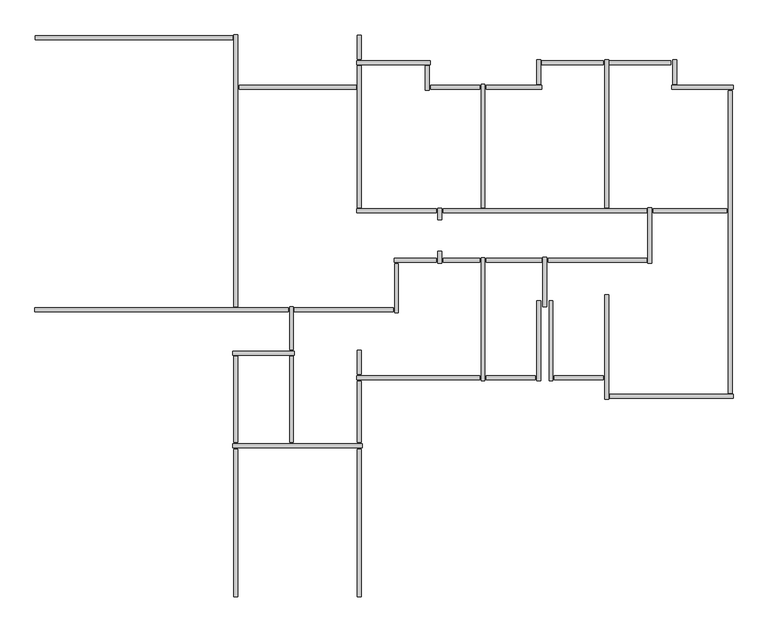
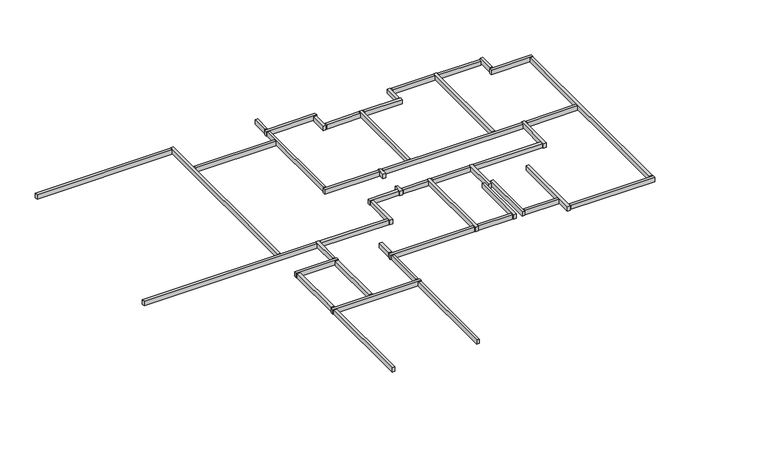
"""IFC4 building model written with IfcOpenShell, lengths in millimetres: beam geometry, Graute viga de respaldo21 : Graute viga de respaldo."""

from ifc_helpers import new_model, si_unit, frame, origin, place, context, project, spatial, polyline, outline, extrude, source, transform, mapped, element, save


def beam_0cd8a0a3(model_context):
    return source(origin(), model_context, "Body", "SweptSolid", [
        extrude(outline(polyline([(-62804.9587292, 72814.9577736), (-62804.9587292, 72720.9577736), (-67594.9587292, 72720.9577736), (-67594.9587292, 72814.9577736), (-62804.9587292, 72814.9577736)])), frame((0.0, 0.0, 17632.9999999), z_axis=(0.0, 0.0, 1.0), x_axis=(1.0, 0.0, 0.0)), (0.0, 0.0, 1.0), 167.0),
        extrude(outline(polyline([(-59771.9587292, 62785.4278788), (-59677.9587292, 62785.4278788), (-59677.9587292, 59195.4278788), (-59771.9587292, 59195.4278788), (-59771.9587292, 62785.4278788)])), frame((0.0, 0.0, 17632.9999999), z_axis=(0.0, 0.0, 1.0), x_axis=(1.0, 0.0, 0.0)), (0.0, 0.0, 1.0), 167.0),
        extrude(outline(polyline([(-62771.9587292, 62785.4278788), (-62677.9587292, 62785.4278788), (-62677.9587292, 59195.4278788), (-62771.9587292, 59195.4278788), (-62771.9587292, 62785.4278788)])), frame((0.0, 0.0, 17632.9999999), z_axis=(0.0, 0.0, 1.0), x_axis=(1.0, 0.0, 0.0)), (0.0, 0.0, 1.0), 167.0),
        extrude(outline(polyline([(-54994.9587292, 64468.4278788), (-54994.9587292, 64562.4278788), (-53804.9587292, 64562.4278788), (-53804.9587292, 64468.4278788), (-54994.9587292, 64468.4278788)])), frame((0.0, 0.0, 17632.9999999), z_axis=(0.0, 0.0, 1.0), x_axis=(1.0, 0.0, 0.0)), (0.0, 0.0, 1.0), 167.0),
        extrude(outline(polyline([(-56644.9587292, 64468.4278788), (-56644.9587292, 64562.4278788), (-55454.9587292, 64562.4278788), (-55454.9587292, 64468.4278788), (-56644.9587292, 64468.4278788)])), frame((0.0, 0.0, 17632.9999999), z_axis=(0.0, 0.0, 1.0), x_axis=(1.0, 0.0, 0.0)), (0.0, 0.0, 1.0), 167.0),
        extrude(outline(polyline([(-52594.9587292, 68518.4278788), (-52594.9587292, 68612.4278788), (-50804.9587292, 68612.4278788), (-50804.9587292, 68518.4278788), (-52594.9587292, 68518.4278788)])), frame((0.0, 0.0, 17632.9999999), z_axis=(0.0, 0.0, 1.0), x_axis=(1.0, 0.0, 0.0)), (0.0, 0.0, 1.0), 167.0),
        extrude(outline(polyline([(-57994.9587292, 71518.4278788), (-57994.9587292, 71612.4278788), (-56804.9587292, 71612.4278788), (-56804.9587292, 71518.4278788), (-57994.9587292, 71518.4278788)])), frame((0.0, 0.0, 17632.9999999), z_axis=(0.0, 0.0, 1.0), x_axis=(1.0, 0.0, 0.0)), (0.0, 0.0, 1.0), 167.0),
        extrude(outline(polyline([(-58027.9587292, 71495.4278788), (-58121.9587292, 71495.4278788), (-58121.9587292, 72085.4278788), (-58027.9587292, 72085.4278788), (-58027.9587292, 71495.4278788)])), frame((0.0, 0.0, 17632.9999999), z_axis=(0.0, 0.0, 1.0), x_axis=(1.0, 0.0, 0.0)), (0.0, 0.0, 1.0), 167.0),
        extrude(outline(polyline([(-59794.9587292, 72118.4278788), (-59794.9587292, 72212.4278788), (-58004.9587292, 72212.4278788), (-58004.9587292, 72118.4278788), (-59794.9587292, 72118.4278788)])), frame((0.0, 0.0, 17632.9999999), z_axis=(0.0, 0.0, 1.0), x_axis=(1.0, 0.0, 0.0)), (0.0, 0.0, 1.0), 167.0),
        extrude(outline(polyline([(-57821.9587292, 68635.4278788), (-57727.9587292, 68635.4278788), (-57727.9587292, 68345.4278788), (-57821.9587292, 68345.4278788), (-57821.9587292, 68635.4278788)])), frame((0.0, 0.0, 17632.9999999), z_axis=(0.0, 0.0, 1.0), x_axis=(1.0, 0.0, 0.0)), (0.0, 0.0, 1.0), 167.0),
        extrude(outline(polyline([(-55144.9587292, 67318.4278788), (-55144.9587292, 67412.4278788), (-52754.9587292, 67412.4278788), (-52754.9587292, 67318.4278788), (-55144.9587292, 67318.4278788)])), frame((0.0, 0.0, 17632.9999999), z_axis=(0.0, 0.0, 1.0), x_axis=(1.0, 0.0, 0.0)), (0.0, 0.0, 1.0), 167.0),
        extrude(outline(polyline([(-56644.9587292, 67318.4278788), (-56644.9587292, 67412.4278788), (-55304.9587292, 67412.4278788), (-55304.9587292, 67318.4278788), (-56644.9587292, 67318.4278788)])), frame((0.0, 0.0, 17632.9999999), z_axis=(0.0, 0.0, 1.0), x_axis=(1.0, 0.0, 0.0)), (0.0, 0.0, 1.0), 167.0),
        extrude(outline(polyline([(-57694.9587292, 67318.4278788), (-57694.9587292, 67412.4278788), (-56804.9587292, 67412.4278788), (-56804.9587292, 67318.4278788), (-57694.9587292, 67318.4278788)])), frame((0.0, 0.0, 17632.9999999), z_axis=(0.0, 0.0, 1.0), x_axis=(1.0, 0.0, 0.0)), (0.0, 0.0, 1.0), 167.0),
        extrude(outline(polyline([(-57821.9587292, 67585.4278788), (-57727.9587292, 67585.4278788), (-57727.9587292, 67295.4278788), (-57821.9587292, 67295.4278788), (-57821.9587292, 67585.4278788)])), frame((0.0, 0.0, 17632.9999999), z_axis=(0.0, 0.0, 1.0), x_axis=(1.0, 0.0, 0.0)), (0.0, 0.0, 1.0), 167.0),
        extrude(outline(polyline([(-58884.9587292, 67318.4278788), (-58884.9587292, 67412.4278788), (-57854.9587292, 67412.4278788), (-57854.9587292, 67318.4278788), (-58884.9587292, 67318.4278788)])), frame((0.0, 0.0, 17632.9999999), z_axis=(0.0, 0.0, 1.0), x_axis=(1.0, 0.0, 0.0)), (0.0, 0.0, 1.0), 167.0),
        extrude(outline(polyline([(-58777.9587292, 66095.4278788), (-58871.9587292, 66095.4278788), (-58871.9587292, 67285.4278788), (-58777.9587292, 67285.4278788), (-58777.9587292, 66095.4278788)])), frame((0.0, 0.0, 17632.9999999), z_axis=(0.0, 0.0, 1.0), x_axis=(1.0, 0.0, 0.0)), (0.0, 0.0, 1.0), 167.0),
        extrude(outline(polyline([(-61304.9587292, 66118.4278788), (-61304.9587292, 66212.4278788), (-58904.9587292, 66212.4278788), (-58904.9587292, 66118.4278788), (-61304.9587292, 66118.4278788)])), frame((0.0, 0.0, 17632.9999999), z_axis=(0.0, 0.0, 1.0), x_axis=(1.0, 0.0, 0.0)), (0.0, 0.0, 1.0), 167.0),
        extrude(outline(polyline([(-56771.9587292, 67430.4278788), (-56677.9587292, 67430.4278788), (-56677.9587292, 64445.4278788), (-56771.9587292, 64445.4278788), (-56771.9587292, 67430.4278788)])), frame((0.0, 0.0, 17632.9999999), z_axis=(0.0, 0.0, 1.0), x_axis=(1.0, 0.0, 0.0)), (0.0, 0.0, 1.0), 167.0),
        extrude(outline(polyline([(-59794.9587292, 64468.4278788), (-59794.9587292, 64562.4278788), (-56804.9587292, 64562.4278788), (-56804.9587292, 64468.4278788), (-59794.9587292, 64468.4278788)])), frame((0.0, 0.0, 17632.9999999), z_axis=(0.0, 0.0, 1.0), x_axis=(1.0, 0.0, 0.0)), (0.0, 0.0, 1.0), 167.0),
        extrude(outline(polyline([(-59771.9587292, 65185.4278788), (-59677.9587292, 65185.4278788), (-59677.9587292, 64595.4278788), (-59771.9587292, 64595.4278788), (-59771.9587292, 65185.4278788)])), frame((0.0, 0.0, 17632.9999999), z_axis=(0.0, 0.0, 1.0), x_axis=(1.0, 0.0, 0.0)), (0.0, 0.0, 1.0), 167.0),
        extrude(outline(polyline([(-59677.9587292, 62945.4278788), (-59771.9587292, 62945.4278788), (-59771.9587292, 64435.4278788), (-59677.9587292, 64435.4278788), (-59677.9587292, 62945.4278788)])), frame((0.0, 0.0, 17632.9999999), z_axis=(0.0, 0.0, 1.0), x_axis=(1.0, 0.0, 0.0)), (0.0, 0.0, 1.0), 167.0),
        extrude(outline(polyline([(-62677.9587292, 62945.4278788), (-62771.9587292, 62945.4278788), (-62771.9587292, 65035.4278788), (-62677.9587292, 65035.4278788), (-62677.9587292, 62945.4278788)])), frame((0.0, 0.0, 17632.9999999), z_axis=(0.0, 0.0, 1.0), x_axis=(1.0, 0.0, 0.0)), (0.0, 0.0, 1.0), 167.0),
        extrude(outline(polyline([(-61327.9587292, 62945.4278788), (-61421.9587292, 62945.4278788), (-61421.9587292, 65035.4278788), (-61327.9587292, 65035.4278788), (-61327.9587292, 62945.4278788)])), frame((0.0, 0.0, 17632.9999999), z_axis=(0.0, 0.0, 1.0), x_axis=(1.0, 0.0, 0.0)), (0.0, 0.0, 1.0), 167.0),
        extrude(outline(polyline([(-61421.9587292, 66235.4278788), (-61327.9587292, 66235.4278788), (-61327.9587292, 65195.4278788), (-61421.9587292, 65195.4278788), (-61421.9587292, 66235.4278788)])), frame((0.0, 0.0, 17632.9999999), z_axis=(0.0, 0.0, 1.0), x_axis=(1.0, 0.0, 0.0)), (0.0, 0.0, 1.0), 167.0),
        extrude(outline(polyline([(-62644.9587292, 71518.4278788), (-62644.9587292, 71612.4278788), (-59804.9587292, 71612.4278788), (-59804.9587292, 71518.4278788), (-62644.9587292, 71518.4278788)])), frame((0.0, 0.0, 17632.9999999), z_axis=(0.0, 0.0, 1.0), x_axis=(1.0, 0.0, 0.0)), (0.0, 0.0, 1.0), 167.0),
        extrude(outline(polyline([(-59677.9587292, 68645.4278788), (-59771.9587292, 68645.4278788), (-59771.9587292, 72085.4278788), (-59677.9587292, 72085.4278788), (-59677.9587292, 68645.4278788)])), frame((0.0, 0.0, 17632.9999999), z_axis=(0.0, 0.0, 1.0), x_axis=(1.0, 0.0, 0.0)), (0.0, 0.0, 1.0), 167.0),
        extrude(outline(polyline([(-59794.9587292, 68518.4278788), (-59794.9587292, 68612.4278788), (-57854.9587292, 68612.4278788), (-57854.9587292, 68518.4278788), (-59794.9587292, 68518.4278788)])), frame((0.0, 0.0, 17632.9999999), z_axis=(0.0, 0.0, 1.0), x_axis=(1.0, 0.0, 0.0)), (0.0, 0.0, 1.0), 167.0),
        extrude(outline(polyline([(-57694.9587292, 68518.4278788), (-57694.9587292, 68612.4278788), (-52754.9587292, 68612.4278788), (-52754.9587292, 68518.4278788), (-57694.9587292, 68518.4278788)])), frame((0.0, 0.0, 17632.9999999), z_axis=(0.0, 0.0, 1.0), x_axis=(1.0, 0.0, 0.0)), (0.0, 0.0, 1.0), 167.0),
        extrude(outline(polyline([(-56771.9587292, 71635.4278788), (-56677.9587292, 71635.4278788), (-56677.9587292, 68645.4278788), (-56771.9587292, 68645.4278788), (-56771.9587292, 71635.4278788)])), frame((0.0, 0.0, 17632.9999999), z_axis=(0.0, 0.0, 1.0), x_axis=(1.0, 0.0, 0.0)), (0.0, 0.0, 1.0), 167.0),
        extrude(outline(polyline([(-55304.9587292, 71612.4278788), (-55304.9587292, 71518.4278788), (-56644.9587292, 71518.4278788), (-56644.9587292, 71612.4278788), (-55304.9587292, 71612.4278788)])), frame((0.0, 0.0, 17632.9999999), z_axis=(0.0, 0.0, 1.0), x_axis=(1.0, 0.0, 0.0)), (0.0, 0.0, 1.0), 167.0),
        extrude(outline(polyline([(-55421.9587292, 72235.4278788), (-55327.9587292, 72235.4278788), (-55327.9587292, 71645.4278788), (-55421.9587292, 71645.4278788), (-55421.9587292, 72235.4278788)])), frame((0.0, 0.0, 17632.9999999), z_axis=(0.0, 0.0, 1.0), x_axis=(1.0, 0.0, 0.0)), (0.0, 0.0, 1.0), 167.0),
        extrude(outline(polyline([(-55294.9587292, 72118.4278788), (-55294.9587292, 72212.4278788), (-53804.9587292, 72212.4278788), (-53804.9587292, 72118.4278788), (-55294.9587292, 72118.4278788)])), frame((0.0, 0.0, 17632.9999999), z_axis=(0.0, 0.0, 1.0), x_axis=(1.0, 0.0, 0.0)), (0.0, 0.0, 1.0), 167.0),
        extrude(outline(polyline([(-52165.9809043, 72212.4278788), (-52165.9809043, 72117.4278788), (-53654.9587292, 72117.4278788), (-53654.9587292, 72212.4278788), (-52165.9809043, 72212.4278788)])), frame((0.0, 0.0, 17617.1856208), z_axis=(0.0, 0.0, 1.0), x_axis=(1.0, 0.0, 0.0)), (0.0, 0.0, 1.0), 165.0),
        extrude(outline(polyline([(-50677.9587292, 64145.4278788), (-50771.9587292, 64145.4278788), (-50771.9587292, 71485.4278788), (-50677.9587292, 71485.4278788), (-50677.9587292, 64145.4278788)])), frame((0.0, 0.0, 17632.9999999), z_axis=(0.0, 0.0, 1.0), x_axis=(1.0, 0.0, 0.0)), (0.0, 0.0, 1.0), 167.0),
        extrude(outline(polyline([(-52627.9587292, 67295.4278788), (-52721.9587292, 67295.4278788), (-52721.9587292, 68640.7810915), (-52627.9587292, 68640.7810915), (-52627.9587292, 67295.4278788)])), frame((0.0, 0.0, 17632.9999999), z_axis=(0.0, 0.0, 1.0), x_axis=(1.0, 0.0, 0.0)), (0.0, 0.0, 1.0), 167.0),
        extrude(outline(polyline([(-55177.9587292, 66245.4278788), (-55271.9587292, 66245.4278788), (-55271.9587292, 67435.4278788), (-55177.9587292, 67435.4278788), (-55177.9587292, 66245.4278788)])), frame((0.0, 0.0, 17632.9999999), z_axis=(0.0, 0.0, 1.0), x_axis=(1.0, 0.0, 0.0)), (0.0, 0.0, 1.0), 167.0),
        extrude(outline(polyline([(-55027.9587292, 64445.4278788), (-55121.9587292, 64445.4278788), (-55121.9587292, 66385.4278788), (-55027.9587292, 66385.4278788), (-55027.9587292, 64445.4278788)])), frame((0.0, 0.0, 17632.9999999), z_axis=(0.0, 0.0, 1.0), x_axis=(1.0, 0.0, 0.0)), (0.0, 0.0, 1.0), 167.0),
        extrude(outline(polyline([(-55327.9587292, 64445.4278788), (-55421.9587292, 64445.4278788), (-55421.9587292, 66385.4278788), (-55327.9587292, 66385.4278788), (-55327.9587292, 64445.4278788)])), frame((0.0, 0.0, 17632.9999999), z_axis=(0.0, 0.0, 1.0), x_axis=(1.0, 0.0, 0.0)), (0.0, 0.0, 1.0), 167.0),
        extrude(outline(polyline([(-53677.9587292, 63995.4278788), (-53771.9587292, 63995.4278788), (-53771.9587292, 66535.4278788), (-53677.9587292, 66535.4278788), (-53677.9587292, 63995.4278788)])), frame((0.0, 0.0, 17632.9999999), z_axis=(0.0, 0.0, 1.0), x_axis=(1.0, 0.0, 0.0)), (0.0, 0.0, 1.0), 167.0),
        extrude(outline(polyline([(-50654.9587292, 64112.4278788), (-50654.9587292, 64018.4278788), (-53644.9587292, 64018.4278788), (-53644.9587292, 64112.4278788), (-50654.9587292, 64112.4278788)])), frame((0.0, 0.0, 17632.9999999), z_axis=(0.0, 0.0, 1.0), x_axis=(1.0, 0.0, 0.0)), (0.0, 0.0, 1.0), 167.0),
        extrude(outline(polyline([(-52121.9587292, 72235.4278788), (-52027.9587292, 72235.4278788), (-52027.9587292, 71645.4278788), (-52121.9587292, 71645.4278788), (-52121.9587292, 72235.4278788)])), frame((0.0, 0.0, 17632.9999999), z_axis=(0.0, 0.0, 1.0), x_axis=(1.0, 0.0, 0.0)), (0.0, 0.0, 1.0), 167.0),
        extrude(outline(polyline([(-52144.9587292, 71518.4278788), (-52144.9587292, 71612.4278788), (-50654.9587292, 71612.4278788), (-50654.9587292, 71518.4278788), (-52144.9587292, 71518.4278788)])), frame((0.0, 0.0, 17632.9999999), z_axis=(0.0, 0.0, 1.0), x_axis=(1.0, 0.0, 0.0)), (0.0, 0.0, 1.0), 167.0),
        extrude(outline(polyline([(-53771.9587292, 72235.4278788), (-53677.9587292, 72235.4278788), (-53677.9587292, 68645.4278788), (-53771.9587292, 68645.4278788), (-53771.9587292, 72235.4278788)])), frame((0.0, 0.0, 17632.9999999), z_axis=(0.0, 0.0, 1.0), x_axis=(1.0, 0.0, 0.0)), (0.0, 0.0, 1.0), 167.0),
        extrude(outline(polyline([(-59771.9587292, 72835.4278788), (-59677.9587292, 72835.4278788), (-59677.9587292, 72245.4278788), (-59771.9587292, 72245.4278788), (-59771.9587292, 72835.4278788)])), frame((0.0, 0.0, 17632.9999999), z_axis=(0.0, 0.0, 1.0), x_axis=(1.0, 0.0, 0.0)), (0.0, 0.0, 1.0), 167.0),
        extrude(outline(polyline([(-62794.9587292, 65068.4278788), (-62794.9587292, 65162.4278788), (-61304.9587292, 65162.4278788), (-61304.9587292, 65068.4278788), (-62794.9587292, 65068.4278788)])), frame((0.0, 0.0, 17632.9999999), z_axis=(0.0, 0.0, 1.0), x_axis=(1.0, 0.0, 0.0)), (0.0, 0.0, 1.0), 167.0),
        extrude(outline(polyline([(-62794.9587292, 62818.4278788), (-62794.9587292, 62912.4278788), (-59654.9587292, 62912.4278788), (-59654.9587292, 62818.4278788), (-62794.9587292, 62818.4278788)])), frame((0.0, 0.0, 17632.9999999), z_axis=(0.0, 0.0, 1.0), x_axis=(1.0, 0.0, 0.0)), (0.0, 0.0, 1.0), 167.0),
        extrude(outline(polyline([(-67601.7587292, 66118.4278788), (-67601.7587292, 66212.4278788), (-61454.9587292, 66212.4278788), (-61454.9587292, 66118.4278788), (-67601.7587292, 66118.4278788)])), frame((0.0, 0.0, 17632.9999999), z_axis=(0.0, 0.0, 1.0), x_axis=(1.0, 0.0, 0.0)), (0.0, 0.0, 1.0), 167.0),
        extrude(outline(polyline([(-62771.9587292, 72837.9577736), (-62677.9587292, 72837.9577736), (-62677.9587292, 66245.4278788), (-62771.9587292, 66245.4278788), (-62771.9587292, 72837.9577736)])), frame((0.0, 0.0, 17632.9999999), z_axis=(0.0, 0.0, 1.0), x_axis=(1.0, 0.0, 0.0)), (0.0, 0.0, 1.0), 167.0),
    ])


if __name__ == "__main__":
    model = new_model("IFC4")
    model_context = context("Model", 3, world=origin())
    ifc_project = project(units=[si_unit("LENGTHUNIT", "METRE", prefix="MILLI")], contexts=[model_context])
    site = spatial("IfcSite", under=ifc_project)
    building = spatial("IfcBuilding", under=site)
    placement = place(None, origin())
    beam_shape = beam_0cd8a0a3(model_context)
    element("IfcBeam", 1, ObjectType="Graute viga de respaldo21 : Graute viga de respaldo", at=placement, inside=building, context=model_context, shape_type="MappedRepresentation", body=[
        mapped(beam_shape, transform((0.0, 0.0, 0.0), x_axis=(1.0, 0.0, 0.0), y_axis=(0.0, 1.0, 0.0), z_axis=(0.0, 0.0, 1.0))),
    ])
    save(model, "model.ifc")

# Revit data of these elements
# Element 1 (IfcBeam, "Graute viga de respaldo21 : Graute viga de respaldo")
#   Materials on its faces: "Concreto, Faixa de areia/cimento"
# Materials
#   "Concreto, Faixa de areia/cimento": class "Concreto", colour RGB 127 127 127, transparency 0, Description = "Revestimento de laje de concreto", Cost = 0
